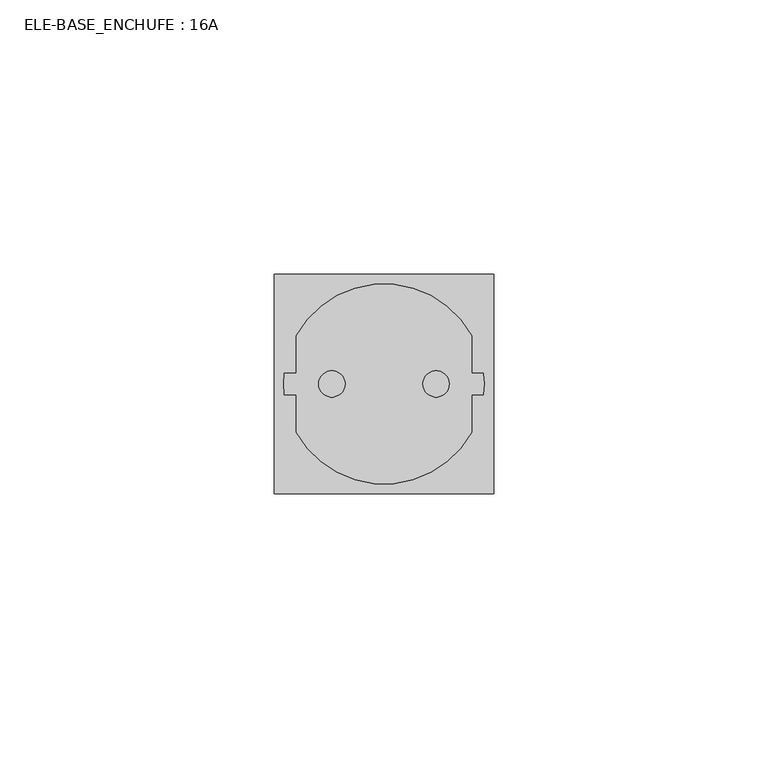
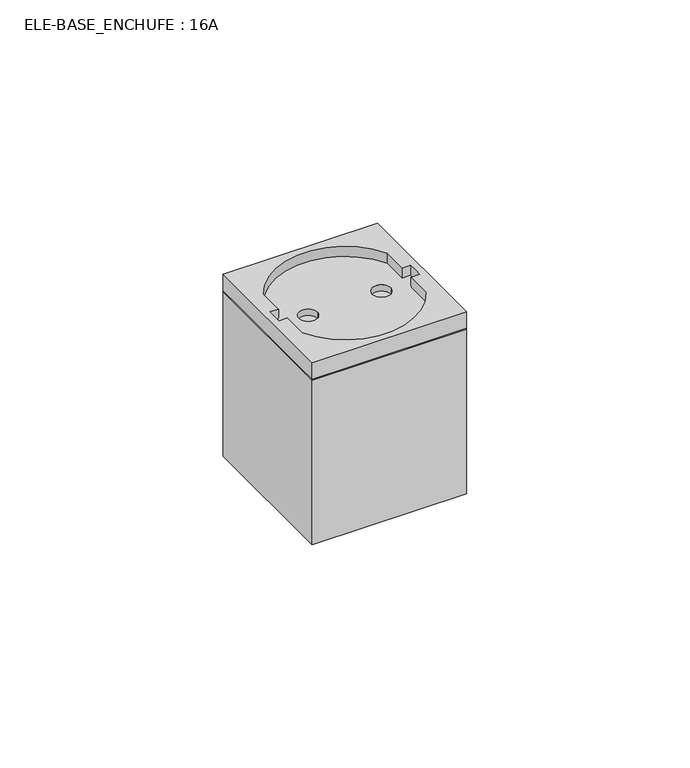
"""IFC4 building model written with IfcOpenShell, lengths in millimetres: proxy geometry, ELE-BASE_ENCHUFE : 16A."""

import ifcopenshell
import ifcopenshell.guid

model = None  # the IFC model being written
_history = None  # IfcOwnerHistory: only IFC2X3 demands one
_inside = {}  # id of a spatial element -> (the spatial element, [elements in it])
_under = {}  # id of a project, library or spatial element -> (it, [spatial elements below it])
_declared = {}  # id of a project -> (the project, [libraries it declares])
_typed = {}  # id of a type object -> (the type object, [elements of that type])
_made_of = {}  # id of a material, layer set ... -> (it, [elements and type objects made of it])


def new_model(schema):
    """Start an empty IFC model of exactly this schema.

    Asked for "IFC4X3", IfcOpenShell would pick the latest addendum, in which some entities
    have other attributes; the version numbers below select the first issue.
    IFC2X3 requires an IfcOwnerHistory on every rooted entity: one is made here for all.
    """
    global model, _history
    if schema == "IFC4X3":
        model = ifcopenshell.file(schema_version=(4, 3, 0, 0))
    else:
        model = ifcopenshell.file(schema=schema)
    _inside.clear()
    _under.clear()
    _declared.clear()
    _typed.clear()
    _made_of.clear()
    _history = None
    if model.schema == "IFC2X3":
        org = make("IfcOrganization", Name="unknown")
        user = make(
            "IfcPersonAndOrganization",
            ThePerson=make("IfcPerson", FamilyName="unknown"),
            TheOrganization=org,
        )
        app = make(
            "IfcApplication",
            ApplicationDeveloper=org,
            Version="unknown",
            ApplicationFullName="unknown",
            ApplicationIdentifier="unknown",
        )
        _history = make(
            "IfcOwnerHistory",
            OwningUser=user,
            OwningApplication=app,
            ChangeAction="ADDED",
            CreationDate=0,
        )
    return model


def make(cls, **values):
    """One entity of the class cls with the attributes given. An attribute that is None is left unset."""
    return model.create_entity(
        cls, **{name: value for name, value in values.items() if value is not None}
    )


def rooted(cls, **values):
    """An entity with a GlobalId (a new one), such as an element, a storey or a relation."""
    return make(cls, GlobalId=ifcopenshell.guid.new(), OwnerHistory=_history, **values)


def si_unit(unit_type, name, prefix=None):
    """IfcSIUnit, for example si_unit("LENGTHUNIT", "METRE", prefix="MILLI")."""
    return make("IfcSIUnit", UnitType=unit_type, Prefix=prefix, Name=name)


def assignment(units):
    """IfcUnitAssignment: the units of a project."""
    return None if units is None else make("IfcUnitAssignment", Units=units)


def point(xyz):
    """IfcCartesianPoint."""
    return None if xyz is None else make("IfcCartesianPoint", Coordinates=xyz)


def direction(xyz):
    """IfcDirection."""
    return None if xyz is None else make("IfcDirection", DirectionRatios=xyz)


def frame(location, z_axis=None, x_axis=None):
    """IfcAxis2Placement3D, a coordinate frame: its origin and axes. An axis left out is left unset."""
    return make(
        "IfcAxis2Placement3D",
        Location=point(location),
        Axis=direction(z_axis),
        RefDirection=direction(x_axis),
    )


def origin():
    """The frame at (0, 0, 0) with its axes left unset."""
    return frame((0.0, 0.0, 0.0))


def place(relative_to, where):
    """IfcLocalPlacement: puts the frame where relative to a parent placement (None: the world)."""
    return make(
        "IfcLocalPlacement", PlacementRelTo=relative_to, RelativePlacement=where
    )


def context(
    kind, dimensions, precision=None, world=None, true_north=None, identifier=None
):
    """IfcGeometricRepresentationContext, for example the 3D "Model" context."""
    return make(
        "IfcGeometricRepresentationContext",
        ContextIdentifier=identifier,
        ContextType=kind,
        CoordinateSpaceDimension=dimensions,
        Precision=precision,
        WorldCoordinateSystem=world,
        TrueNorth=true_north,
    )


def project(units=None, contexts=None):
    """IfcProject with its units and contexts."""
    return rooted(
        "IfcProject",
        Name="project",
        RepresentationContexts=contexts,
        UnitsInContext=assignment(units),
    )


def spatial(cls, under=None, at=None, **own):
    """A site, building, storey or space (cls), placed at a placement, below another one or the project."""
    s = rooted(cls, ObjectPlacement=at, **own)
    if under is not None:
        _under.setdefault(under.id(), (under, []))[1].append(s)
    return s


def polyline(points):
    """IfcPolyline through the points."""
    return make("IfcPolyline", Points=[point(p) for p in points])


def circle_curve(where, radius):
    """IfcCircle in the frame where."""
    return make("IfcCircle", Position=where, Radius=radius)


def outline(outer, holes=None, kind="AREA"):
    """IfcArbitraryClosedProfileDef: a profile drawn as a closed curve; with holes, ...WithVoids."""
    if holes is None:
        return make("IfcArbitraryClosedProfileDef", ProfileType=kind, OuterCurve=outer)
    return make(
        "IfcArbitraryProfileDefWithVoids",
        ProfileType=kind,
        OuterCurve=outer,
        InnerCurves=holes,
    )


def extrude(swept, where, along, depth):
    """IfcExtrudedAreaSolid: the profile swept, set in the frame where, extruded along a direction by depth."""
    return make(
        "IfcExtrudedAreaSolid",
        SweptArea=swept,
        Position=where,
        ExtrudedDirection=direction(along),
        Depth=depth,
    )


def shape(context_of_items, identifier, shape_type, items):
    """IfcShapeRepresentation: the items that make up one representation, for example the "Body"."""
    return make(
        "IfcShapeRepresentation",
        ContextOfItems=context_of_items,
        RepresentationIdentifier=identifier,
        RepresentationType=shape_type,
        Items=items,
    )


def source(mapping_origin, context_of_items, identifier, shape_type, items):
    """IfcRepresentationMap: a shape defined once, which mapped items show again and again."""
    return make(
        "IfcRepresentationMap",
        MappingOrigin=mapping_origin,
        MappedRepresentation=shape(context_of_items, identifier, shape_type, items),
    )


def transform(
    local_origin,
    x_axis=None,
    y_axis=None,
    z_axis=None,
    scale=None,
    scale2=None,
    scale3=None,
    uniform=True,
):
    """IfcCartesianTransformationOperator3D, or its non-uniform kind. x_axis, y_axis, z_axis: its Axis1, 2, 3."""
    if uniform:
        return make(
            "IfcCartesianTransformationOperator3D",
            Axis1=direction(x_axis),
            Axis2=direction(y_axis),
            LocalOrigin=point(local_origin),
            Scale=scale,
            Axis3=direction(z_axis),
        )
    return make(
        "IfcCartesianTransformationOperator3DnonUniform",
        Axis1=direction(x_axis),
        Axis2=direction(y_axis),
        LocalOrigin=point(local_origin),
        Scale=scale,
        Axis3=direction(z_axis),
        Scale2=scale2,
        Scale3=scale3,
    )


def mapped(mapping_source, mapping_target):
    """IfcMappedItem: shows the shape of a source again, moved by a transform."""
    return make(
        "IfcMappedItem", MappingSource=mapping_source, MappingTarget=mapping_target
    )


def made_of(thing, what):
    """Note that an element or type object is made of a material, layer set ...; save() writes the relation."""
    if what is not None:
        _made_of.setdefault(what.id(), (what, []))[1].append(thing)
    return thing


def element(
    cls,
    number,
    at=None,
    inside=None,
    cuts=None,
    type_object=None,
    material=None,
    context=None,
    identifier="Body",
    shape_type=None,
    held_by="IfcProductDefinitionShape",
    body=None,
    shapes=None,
    **own,
):
    """One element of the class cls, such as IfcWall. Its Tag is "e" and its number.

    at: its placement. inside: the storey or other place that contains it. cuts: it is an
    opening in that element (IfcRelVoidsElement). A single representation is given by context,
    identifier, shape_type and body (its items); several are given by shapes. held_by: the class
    of the entity that holds the representations. save() writes the other relations.
    """
    e = rooted(cls, Tag="e%d" % number, ObjectPlacement=at, **own)
    if body is not None:
        shapes = [shape(context, identifier, shape_type, body)]
    if shapes is not None:
        e.Representation = make(held_by, Representations=shapes)
    if inside is not None:
        _inside.setdefault(inside.id(), (inside, []))[1].append(e)
    if cuts is not None:
        rooted(
            "IfcRelVoidsElement", RelatingBuildingElement=cuts, RelatedOpeningElement=e
        )
    if type_object is not None:
        _typed.setdefault(type_object.id(), (type_object, []))[1].append(e)
    return made_of(e, material)


def aggregate(whole, parts):
    """IfcRelAggregates: a whole, such as a stair, and the parts it consists of."""
    return rooted("IfcRelAggregates", RelatingObject=whole, RelatedObjects=parts)


def save(model, path):
    """Write the relations noted so far, then the file.

    IfcRelAggregates (storeys below a building ...), IfcRelContainedInSpatialStructure (elements
    in a storey), IfcRelDefinesByType, IfcRelAssociatesMaterial and IfcRelDeclares: one each for
    every whole, place, type object, material and project.
    """
    for whole, parts in _under.values():
        aggregate(whole, parts)
    for where, things in _inside.values():
        rooted(
            "IfcRelContainedInSpatialStructure",
            RelatedElements=things,
            RelatingStructure=where,
        )
    for kind, things in _typed.values():
        rooted("IfcRelDefinesByType", RelatedObjects=things, RelatingType=kind)
    for what, things in _made_of.values():
        rooted("IfcRelAssociatesMaterial", RelatedObjects=things, RelatingMaterial=what)
    for by, libraries in _declared.values():
        rooted("IfcRelDeclares", RelatingContext=by, RelatedDefinitions=libraries)
    model.write(path)


def plane_surface(at):
    """IfcPlane: the flat surface through the origin of the frame at, square to its z axis."""
    return make("IfcPlane", Position=at)


def revolved_surface(curve, axis_point, axis_direction):
    """IfcSurfaceOfRevolution: the curve turned about the line through axis_point along axis_direction."""
    return make(
        "IfcSurfaceOfRevolution",
        SweptCurve=make("IfcArbitraryOpenProfileDef", ProfileType="CURVE", Curve=curve),
        AxisPosition=make("IfcAxis1Placement", Location=point(axis_point), Axis=direction(axis_direction)),
    )


def advanced_brep(points, edges, surfaces, faces):
    """IfcAdvancedBrep: a solid bounded by faces that lie on surfaces and meet in shared edges.

    An edge is (start, end): straight between two places in points (the first is 0);
    or (start, end, curve); or (start, end, curve, False) where it runs against its curve.
    A face is (place in surfaces, loops), or (place, loops, False) where it looks against
    its surface's normal. A loop lists edges by number (the first is 1), with a minus sign
    where the edge is run from its end to its start. The first loop is the outer one.
    """
    corners = [point(p) for p in points]
    vertices = [make("IfcVertexPoint", VertexGeometry=c) for c in corners]
    made = []
    for start, end, *more in edges:
        made.append(
            make(
                "IfcEdgeCurve",
                EdgeStart=vertices[start],
                EdgeEnd=vertices[end],
                EdgeGeometry=more[0] if more else make("IfcPolyline", Points=[corners[start], corners[end]]),
                SameSense=more[1] if len(more) > 1 else True,
            )
        )
    hull = []
    for where, loops, *sense in faces:
        bounds = []
        for j, loop in enumerate(loops):
            ring = [make("IfcOrientedEdge", EdgeElement=made[abs(k) - 1], Orientation=k > 0) for k in loop]
            bounds.append(
                make(
                    "IfcFaceOuterBound" if j == 0 else "IfcFaceBound",
                    Bound=make("IfcEdgeLoop", EdgeList=ring),
                    Orientation=True,
                )
            )
        hull.append(make("IfcAdvancedFace", Bounds=bounds, FaceSurface=surfaces[where], SameSense=sense[0] if sense else True))
    return make("IfcAdvancedBrep", Outer=make("IfcClosedShell", CfsFaces=hull))


def ele_base_enchufe_16a_49acce93(model_context):
    return source(origin(), model_context, "Body", "SolidModel", [
        extrude(outline(polyline([(20.0, -20.0), (-20.0, -20.0), (-20.0, 20.0), (20.0, 20.0), (20.0, -20.0)])), frame((0.0, 0.0, -45.0), z_axis=(0.0, 0.0, 1.0), x_axis=(1.0, 0.0, 0.0)), (0.0, 0.0, 1.0), 45.0),
        advanced_brep(
        [(20.0, -20.0, 4.7625), (20.0, 20.0, 4.7625), (-20.0, 20.0, 4.7625), (-20.0, -20.0, 4.7625), (-16.0, 8.7785249, 4.7625), (16.0, 8.7785249, 4.7625), (16.0, 2.0, 4.7625), (18.1400799, 2.0, 4.7625), (18.1400799, -2.0, 4.7625), (16.0, -2.0, 4.7625), (16.0, -8.7785249, 4.7625), (-16.0, -8.7785249, 4.7625), (-16.0, -2.0, 4.7625), (-18.1400799, -2.0, 4.7625), (-18.1400799, 2.0, 4.7625), (-16.0, 2.0, 4.7625), (20.0, -20.0, 0.0), (-20.0, -20.0, 0.0), (-20.0, 20.0, 0.0), (20.0, 20.0, 0.0), (-11.9, 0.0, 0.0), (-7.1, 0.0, 0.0), (7.1, 0.0, 0.0), (11.9, 0.0, 0.0), (-16.0, 2.0, 2.0), (-18.1400799, 2.0, 2.0), (-18.1400799, -2.0, 2.0), (-16.0, -2.0, 2.0), (-16.0, -8.7785249, 2.0), (16.0, -8.7785249, 2.0), (16.0, -2.0, 2.0), (18.1400799, -2.0, 2.0), (18.1400799, 2.0, 2.0), (16.0, 2.0, 2.0), (16.0, 8.7785249, 2.0), (-16.0, 8.7785249, 2.0), (-7.1, 0.0, 2.0), (-11.9, 0.0, 2.0), (11.9, 0.0, 2.0), (7.1, 0.0, 2.0)],
        [
            (0, 1),
            (1, 2),
            (2, 3),
            (3, 0),
            (4, 5, circle_curve(frame((0.0, 0.0, 4.7625), z_axis=(0.0, 0.0, -1.0), x_axis=(1.0, 0.0, 0.0)), 18.25)),
            (5, 6),
            (6, 7),
            (7, 8, circle_curve(frame((0.0, 0.0, 4.7625), z_axis=(0.0, 0.0, -1.0), x_axis=(1.0, 0.0, 0.0)), 18.25)),
            (8, 9),
            (9, 10),
            (10, 11, circle_curve(frame((0.0, 0.0, 4.7625), z_axis=(0.0, 0.0, -1.0), x_axis=(1.0, 0.0, 0.0)), 18.25)),
            (11, 12),
            (12, 13),
            (13, 14, circle_curve(frame((0.0, 0.0, 4.7625), z_axis=(0.0, 0.0, -1.0), x_axis=(1.0, 0.0, 0.0)), 18.25)),
            (14, 15),
            (15, 4),
            (16, 17),
            (17, 18),
            (18, 19),
            (19, 16),
            (20, 21, circle_curve(frame((-9.5, 0.0, 0.0), z_axis=(0.0, 0.0, 1.0), x_axis=(1.0, 0.0, 0.0)), 2.4)),
            (21, 20, circle_curve(frame((-9.5, 0.0, 0.0), z_axis=(0.0, 0.0, 1.0), x_axis=(1.0, 0.0, 0.0)), 2.4)),
            (22, 23, circle_curve(frame((9.5, 0.0, 0.0), z_axis=(0.0, 0.0, 1.0), x_axis=(1.0, 0.0, 0.0)), 2.4)),
            (23, 22, circle_curve(frame((9.5, 0.0, 0.0), z_axis=(0.0, 0.0, 1.0), x_axis=(1.0, 0.0, 0.0)), 2.4)),
            (3, 17),
            (16, 0),
            (2, 18),
            (1, 19),
            (24, 25),
            (25, 26, circle_curve(frame((0.0, 0.0, 2.0), z_axis=(0.0, 0.0, 1.0), x_axis=(1.0, 0.0, 0.0)), 18.25)),
            (26, 27),
            (27, 28),
            (28, 29, circle_curve(frame((0.0, 0.0, 2.0), z_axis=(0.0, 0.0, 1.0), x_axis=(1.0, 0.0, 0.0)), 18.25)),
            (29, 30),
            (30, 31),
            (31, 32, circle_curve(frame((0.0, 0.0, 2.0), z_axis=(0.0, 0.0, 1.0), x_axis=(1.0, 0.0, 0.0)), 18.25)),
            (32, 33),
            (33, 34),
            (34, 35, circle_curve(frame((0.0, 0.0, 2.0), z_axis=(0.0, 0.0, 1.0), x_axis=(1.0, 0.0, 0.0)), 18.25)),
            (35, 24),
            (36, 37, circle_curve(frame((-9.5, 0.0, 2.0), z_axis=(0.0, 0.0, -1.0), x_axis=(1.0, 0.0, 0.0)), 2.4)),
            (37, 36, circle_curve(frame((-9.5, 0.0, 2.0), z_axis=(0.0, 0.0, -1.0), x_axis=(1.0, 0.0, 0.0)), 2.4)),
            (38, 39, circle_curve(frame((9.5, 0.0, 2.0), z_axis=(0.0, 0.0, -1.0), x_axis=(1.0, 0.0, 0.0)), 2.4)),
            (39, 38, circle_curve(frame((9.5, 0.0, 2.0), z_axis=(0.0, 0.0, -1.0), x_axis=(1.0, 0.0, 0.0)), 2.4)),
            (35, 4),
            (15, 24),
            (34, 5),
            (33, 6),
            (32, 7),
            (31, 8),
            (30, 9),
            (29, 10),
            (28, 11),
            (27, 12),
            (26, 13),
            (25, 14),
            (21, 36),
            (37, 20),
            (23, 38),
            (39, 22),
        ],
        [
            plane_surface(frame((-40.0, -20.0, 4.7625), z_axis=(0.0, 0.0, 1.0), x_axis=(-1.0, 0.0, 0.0))),
            plane_surface(frame((-40.0, -20.0, 0.0), z_axis=(0.0, 0.0, -1.0), x_axis=(1.0, 0.0, 0.0))),
            plane_surface(frame((20.0, -20.0, 4.7625), z_axis=(0.0, -1.0, 0.0), x_axis=(0.0, 0.0, -1.0))),
            plane_surface(frame((-20.0, -20.0, 4.7625), z_axis=(-1.0, 0.0, 0.0), x_axis=(0.0, 0.0, -1.0))),
            plane_surface(frame((-20.0, 20.0, 4.7625), z_axis=(0.0, 1.0, 0.0), x_axis=(0.0, 0.0, -1.0))),
            plane_surface(frame((20.0, 20.0, 4.7625), z_axis=(1.0, 0.0, 0.0), x_axis=(0.0, 0.0, -1.0))),
            plane_surface(frame((-16.0, 8.7785249, 2.0), z_axis=(0.0, 0.0, 1.0), x_axis=(0.0, -1.0, 0.0))),
            plane_surface(frame((-16.0, 2.0, 4.8), z_axis=(1.0, 0.0, 0.0), x_axis=(0.0, 0.0, -1.0))),
            revolved_surface(polyline([(18.25, 0.0, 4.7625), (18.25, 0.0, 2.0)]), (0.0, 0.0, 2.0), (0.0, 0.0, 1.0)),
            plane_surface(frame((16.0, 8.7785249, 4.8), z_axis=(-1.0, 0.0, 0.0), x_axis=(0.0, 0.0, -1.0))),
            plane_surface(frame((16.0, 2.0, 4.8), z_axis=(0.0, -1.0, 0.0), x_axis=(0.0, 0.0, -1.0))),
            plane_surface(frame((18.1400799, -2.0, 4.8), z_axis=(0.0, 1.0, 0.0), x_axis=(0.0, 0.0, -1.0))),
            plane_surface(frame((16.0, -2.0, 4.8), z_axis=(-1.0, 0.0, 0.0), x_axis=(0.0, 0.0, -1.0))),
            plane_surface(frame((-16.0, -8.7785249, 4.8), z_axis=(1.0, 0.0, 0.0), x_axis=(0.0, 0.0, -1.0))),
            plane_surface(frame((-16.0, -2.0, 4.8), z_axis=(0.0, 1.0, 0.0), x_axis=(0.0, 0.0, -1.0))),
            plane_surface(frame((-18.1400799, 2.0, 4.8), z_axis=(0.0, -1.0, 0.0), x_axis=(0.0, 0.0, -1.0))),
            revolved_surface(polyline([(-7.1, 0.0, 2.0), (-7.1, 0.0, 0.0)]), (-9.5, 0.0, -18.0), (0.0, 0.0, 1.0)),
            revolved_surface(polyline([(11.9, 0.0, 2.0), (11.9, 0.0, 0.0)]), (9.5, 0.0, 0.0), (0.0, 0.0, 1.0)),
        ],
        [
            (0, [[1, 2, 3, 4], [5, 6, 7, 8, 9, 10, 11, 12, 13, 14, 15, 16]]),
            (1, [[17, 18, 19, 20], [21, 22], [23, 24]]),
            (2, [[25, -17, 26, -4]]),
            (3, [[27, -18, -25, -3]]),
            (4, [[28, -19, -27, -2]]),
            (5, [[-26, -20, -28, -1]]),
            (6, [[29, 30, 31, 32, 33, 34, 35, 36, 37, 38, 39, 40], [41, 42], [43, 44]]),
            (7, [[45, -16, 46, -40]]),
            (8, [[47, -5, -45, -39]]),
            (9, [[48, -6, -47, -38]]),
            (10, [[49, -7, -48, -37]]),
            (8, [[50, -8, -49, -36]]),
            (11, [[51, -9, -50, -35]]),
            (12, [[52, -10, -51, -34]]),
            (8, [[53, -11, -52, -33]]),
            (13, [[54, -12, -53, -32]]),
            (14, [[55, -13, -54, -31]]),
            (8, [[56, -14, -55, -30]]),
            (15, [[-46, -15, -56, -29]]),
            (16, [[-22, 57, -42, 58]]),
            (16, [[-41, -57, -21, -58]]),
            (17, [[-24, 59, -44, 60]]),
            (17, [[-43, -59, -23, -60]]),
        ],
    ),
    ])


if __name__ == "__main__":
    model = new_model("IFC4")
    model_context = context("Model", 3, world=origin())
    ifc_project = project(units=[si_unit("LENGTHUNIT", "METRE", prefix="MILLI")], contexts=[model_context])
    site = spatial("IfcSite", under=ifc_project)
    building = spatial("IfcBuilding", under=site)
    placement = place(None, origin())
    ele_base_enchufe_16a_shape = ele_base_enchufe_16a_49acce93(model_context)
    element("IfcBuildingElementProxy", 1, Name="ELE-BASE_ENCHUFE : 16A", ObjectType="ELE-BASE_ENCHUFE : 16A", at=placement, inside=building, context=model_context, shape_type="MappedRepresentation", body=[
        mapped(ele_base_enchufe_16a_shape, transform((0.0, 0.0, 0.0), x_axis=(1.0, 0.0, 0.0), y_axis=(0.0, 1.0, 0.0), z_axis=(0.0, 0.0, 1.0))),
    ])
    save(model, "model.ifc")

# Revit data of these elements
# Type "ELE-BASE_ENCHUFE : 16A"
#   Etiqueta = ""
#   Voltaje toma corriente = 230 V
#   SimboloPosicionVertical [instance default] = 0.05 m
#   SimboloPosicionHorizontal [instance default] = 0.00 m
#   Potencia = 3680 W
#   Intensidad = 16 A
#   Carga = 3680 VA
#   Default Elevation = 0.20 m
#   Altura = 0.20 m
#   Simbolo25A = no
#   Simbolo16AEstanco = no
#   Simbolo16A = yes
#   Clasificación de carga = Toma de corriente
#   Assembly Code = ""
